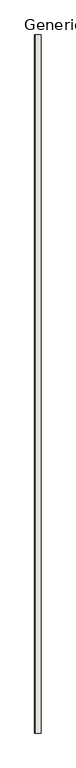
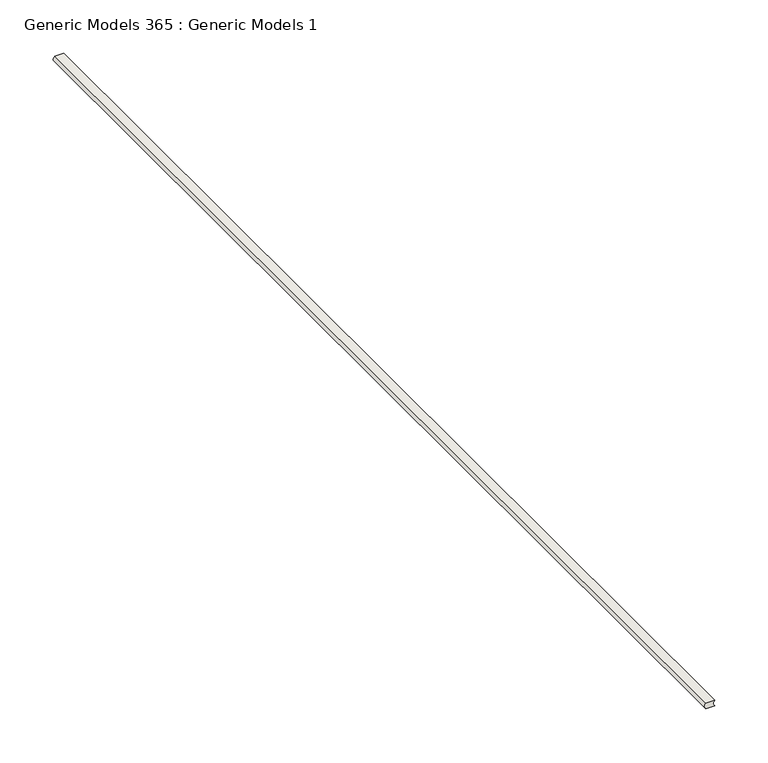
"""IFC4 building model written with IfcOpenShell, lengths in millimetres: wall geometry, Generic Models 365 : Generic Models 1."""

from ifc_helpers import new_model, si_unit, point, frame, frame_2d, origin, place, context, project, spatial, polyline, circle_curve, trimmed, segment, composite_curve, outline, extrude, source, transform, mapped, element, save


def generic_models_365_generic_models_1_292cadf2(model_context):
    return source(origin(), model_context, "Body", "SweptSolid", [
        extrude(outline(composite_curve([segment(polyline([(2457.45, 137582.275), (2457.45, 137572.75)]), True, "CONTINUOUS"), segment(trimmed(circle_curve(frame_2d((2454.275, 137575.6647405)), 4.3100275), [point((2457.45, 137572.75))], [point((2451.1, 137572.75))], False, "CARTESIAN"), True, "CONTINUOUS"), segment(polyline([(2451.1, 137572.75), (2451.1, 137582.275)]), True, "CONTINUOUS"), segment(trimmed(circle_curve(frame_2d((2454.275, 137585.1897405)), 4.3100275), [point((2451.1, 137582.275))], [point((2457.45, 137582.275))], True, "CARTESIAN"), True, "CONTINUOUS")], self_intersect=False)), frame((0.0, 0.0, 0.0), z_axis=(0.0, 1.0, 0.0), x_axis=(0.0, 0.0, 1.0)), (0.0, 0.0, 1.0), 1219.2),
    ])


if __name__ == "__main__":
    model = new_model("IFC4")
    model_context = context("Model", 3, world=origin())
    ifc_project = project(units=[si_unit("LENGTHUNIT", "METRE", prefix="MILLI")], contexts=[model_context])
    site = spatial("IfcSite", under=ifc_project)
    building = spatial("IfcBuilding", under=site)
    placement = place(None, origin())
    generic_models_365_generic_models_1_shape = generic_models_365_generic_models_1_292cadf2(model_context)
    element("IfcWall", 1, ObjectType="Generic Models 365 : Generic Models 1", at=placement, inside=building, context=model_context, shape_type="MappedRepresentation", body=[
        mapped(generic_models_365_generic_models_1_shape, transform((0.0, 0.0, 0.0), x_axis=(1.0, 0.0, 0.0), y_axis=(0.0, 1.0, 0.0), z_axis=(0.0, 0.0, 1.0))),
    ])
    save(model, "model.ifc")

# Revit data of these elements
# Element 1 (IfcWall, "Generic Models 365 : Generic Models 1")
#   Materials on its faces: "CONTINUOUS FIRE RATED SEALANT EACH SIDE."
# Materials
#   "CONTINUOUS FIRE RATED SEALANT EACH SIDE.": class "Miscellaneous", colour RGB 127 127 127, transparency 0, Cost = 0
